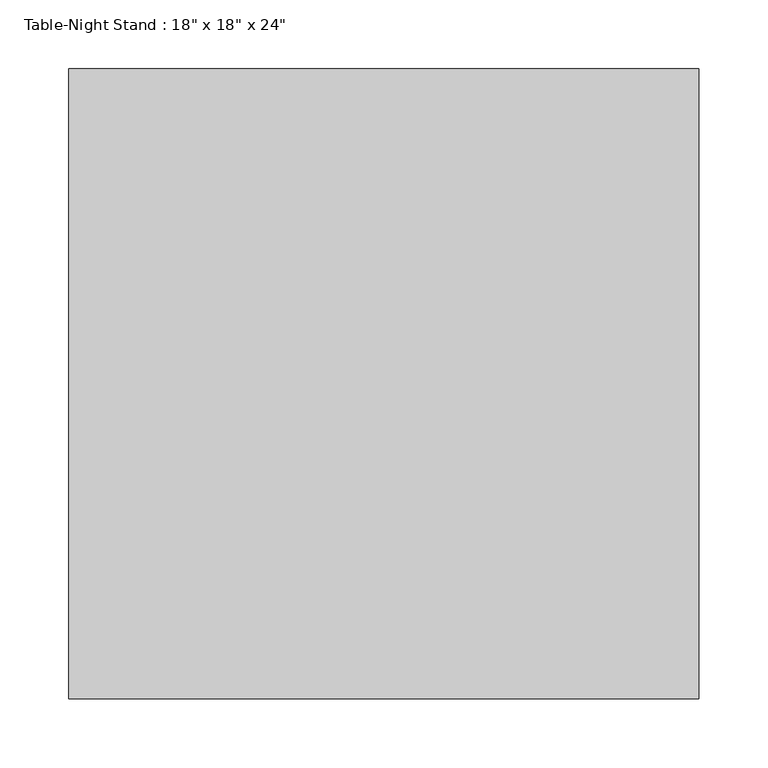
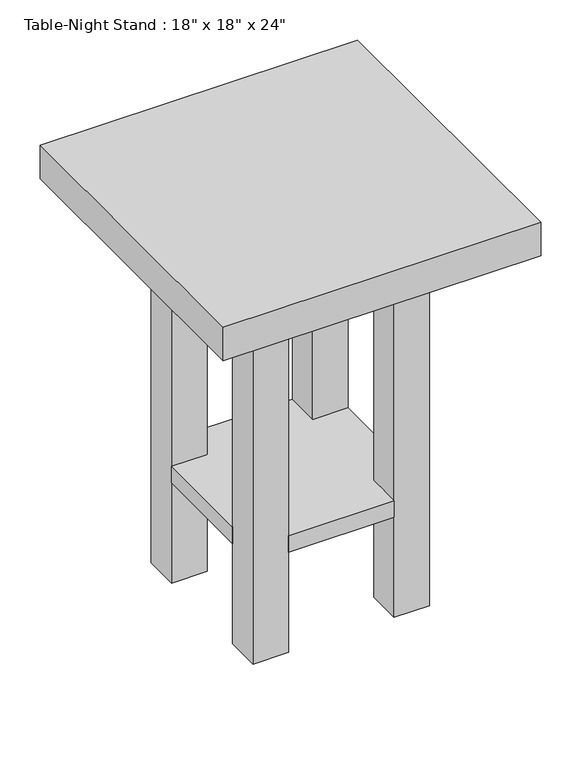
"""IFC4 building model written with IfcOpenShell, lengths in millimetres: furniture geometry."""

import ifcopenshell
import ifcopenshell.guid

model = None  # the IFC model being written
_history = None  # IfcOwnerHistory: only IFC2X3 demands one
_inside = {}  # id of a spatial element -> (the spatial element, [elements in it])
_under = {}  # id of a project, library or spatial element -> (it, [spatial elements below it])
_declared = {}  # id of a project -> (the project, [libraries it declares])
_typed = {}  # id of a type object -> (the type object, [elements of that type])
_made_of = {}  # id of a material, layer set ... -> (it, [elements and type objects made of it])


def new_model(schema):
    """Start an empty IFC model of exactly this schema.

    Asked for "IFC4X3", IfcOpenShell would pick the latest addendum, in which some entities
    have other attributes; the version numbers below select the first issue.
    IFC2X3 requires an IfcOwnerHistory on every rooted entity: one is made here for all.
    """
    global model, _history
    if schema == "IFC4X3":
        model = ifcopenshell.file(schema_version=(4, 3, 0, 0))
    else:
        model = ifcopenshell.file(schema=schema)
    _inside.clear()
    _under.clear()
    _declared.clear()
    _typed.clear()
    _made_of.clear()
    _history = None
    if model.schema == "IFC2X3":
        org = make("IfcOrganization", Name="unknown")
        user = make(
            "IfcPersonAndOrganization",
            ThePerson=make("IfcPerson", FamilyName="unknown"),
            TheOrganization=org,
        )
        app = make(
            "IfcApplication",
            ApplicationDeveloper=org,
            Version="unknown",
            ApplicationFullName="unknown",
            ApplicationIdentifier="unknown",
        )
        _history = make(
            "IfcOwnerHistory",
            OwningUser=user,
            OwningApplication=app,
            ChangeAction="ADDED",
            CreationDate=0,
        )
    return model


def make(cls, **values):
    """One entity of the class cls with the attributes given. An attribute that is None is left unset."""
    return model.create_entity(
        cls, **{name: value for name, value in values.items() if value is not None}
    )


def rooted(cls, **values):
    """An entity with a GlobalId (a new one), such as an element, a storey or a relation."""
    return make(cls, GlobalId=ifcopenshell.guid.new(), OwnerHistory=_history, **values)


def si_unit(unit_type, name, prefix=None):
    """IfcSIUnit, for example si_unit("LENGTHUNIT", "METRE", prefix="MILLI")."""
    return make("IfcSIUnit", UnitType=unit_type, Prefix=prefix, Name=name)


def assignment(units):
    """IfcUnitAssignment: the units of a project."""
    return None if units is None else make("IfcUnitAssignment", Units=units)


def point(xyz):
    """IfcCartesianPoint."""
    return None if xyz is None else make("IfcCartesianPoint", Coordinates=xyz)


def direction(xyz):
    """IfcDirection."""
    return None if xyz is None else make("IfcDirection", DirectionRatios=xyz)


def frame(location, z_axis=None, x_axis=None):
    """IfcAxis2Placement3D, a coordinate frame: its origin and axes. An axis left out is left unset."""
    return make(
        "IfcAxis2Placement3D",
        Location=point(location),
        Axis=direction(z_axis),
        RefDirection=direction(x_axis),
    )


def origin():
    """The frame at (0, 0, 0) with its axes left unset."""
    return frame((0.0, 0.0, 0.0))


def origin_with_axes():
    """The frame at (0, 0, 0) with the z axis (0, 0, 1) and the x axis (1, 0, 0) written out."""
    return frame((0.0, 0.0, 0.0), z_axis=(0.0, 0.0, 1.0), x_axis=(1.0, 0.0, 0.0))


def place(relative_to, where):
    """IfcLocalPlacement: puts the frame where relative to a parent placement (None: the world)."""
    return make(
        "IfcLocalPlacement", PlacementRelTo=relative_to, RelativePlacement=where
    )


def context(
    kind, dimensions, precision=None, world=None, true_north=None, identifier=None
):
    """IfcGeometricRepresentationContext, for example the 3D "Model" context."""
    return make(
        "IfcGeometricRepresentationContext",
        ContextIdentifier=identifier,
        ContextType=kind,
        CoordinateSpaceDimension=dimensions,
        Precision=precision,
        WorldCoordinateSystem=world,
        TrueNorth=true_north,
    )


def project(units=None, contexts=None):
    """IfcProject with its units and contexts."""
    return rooted(
        "IfcProject",
        Name="project",
        RepresentationContexts=contexts,
        UnitsInContext=assignment(units),
    )


def spatial(cls, under=None, at=None, **own):
    """A site, building, storey or space (cls), placed at a placement, below another one or the project."""
    s = rooted(cls, ObjectPlacement=at, **own)
    if under is not None:
        _under.setdefault(under.id(), (under, []))[1].append(s)
    return s


def polyline(points):
    """IfcPolyline through the points."""
    return make("IfcPolyline", Points=[point(p) for p in points])


def outline(outer, holes=None, kind="AREA"):
    """IfcArbitraryClosedProfileDef: a profile drawn as a closed curve; with holes, ...WithVoids."""
    if holes is None:
        return make("IfcArbitraryClosedProfileDef", ProfileType=kind, OuterCurve=outer)
    return make(
        "IfcArbitraryProfileDefWithVoids",
        ProfileType=kind,
        OuterCurve=outer,
        InnerCurves=holes,
    )


def extrude(swept, where, along, depth):
    """IfcExtrudedAreaSolid: the profile swept, set in the frame where, extruded along a direction by depth."""
    return make(
        "IfcExtrudedAreaSolid",
        SweptArea=swept,
        Position=where,
        ExtrudedDirection=direction(along),
        Depth=depth,
    )


def shape(context_of_items, identifier, shape_type, items):
    """IfcShapeRepresentation: the items that make up one representation, for example the "Body"."""
    return make(
        "IfcShapeRepresentation",
        ContextOfItems=context_of_items,
        RepresentationIdentifier=identifier,
        RepresentationType=shape_type,
        Items=items,
    )


def source(mapping_origin, context_of_items, identifier, shape_type, items):
    """IfcRepresentationMap: a shape defined once, which mapped items show again and again."""
    return make(
        "IfcRepresentationMap",
        MappingOrigin=mapping_origin,
        MappedRepresentation=shape(context_of_items, identifier, shape_type, items),
    )


def transform(
    local_origin,
    x_axis=None,
    y_axis=None,
    z_axis=None,
    scale=None,
    scale2=None,
    scale3=None,
    uniform=True,
):
    """IfcCartesianTransformationOperator3D, or its non-uniform kind. x_axis, y_axis, z_axis: its Axis1, 2, 3."""
    if uniform:
        return make(
            "IfcCartesianTransformationOperator3D",
            Axis1=direction(x_axis),
            Axis2=direction(y_axis),
            LocalOrigin=point(local_origin),
            Scale=scale,
            Axis3=direction(z_axis),
        )
    return make(
        "IfcCartesianTransformationOperator3DnonUniform",
        Axis1=direction(x_axis),
        Axis2=direction(y_axis),
        LocalOrigin=point(local_origin),
        Scale=scale,
        Axis3=direction(z_axis),
        Scale2=scale2,
        Scale3=scale3,
    )


def mapped(mapping_source, mapping_target):
    """IfcMappedItem: shows the shape of a source again, moved by a transform."""
    return make(
        "IfcMappedItem", MappingSource=mapping_source, MappingTarget=mapping_target
    )


def made_of(thing, what):
    """Note that an element or type object is made of a material, layer set ...; save() writes the relation."""
    if what is not None:
        _made_of.setdefault(what.id(), (what, []))[1].append(thing)
    return thing


def element(
    cls,
    number,
    at=None,
    inside=None,
    cuts=None,
    type_object=None,
    material=None,
    context=None,
    identifier="Body",
    shape_type=None,
    held_by="IfcProductDefinitionShape",
    body=None,
    shapes=None,
    **own,
):
    """One element of the class cls, such as IfcWall. Its Tag is "e" and its number.

    at: its placement. inside: the storey or other place that contains it. cuts: it is an
    opening in that element (IfcRelVoidsElement). A single representation is given by context,
    identifier, shape_type and body (its items); several are given by shapes. held_by: the class
    of the entity that holds the representations. save() writes the other relations.
    """
    e = rooted(cls, Tag="e%d" % number, ObjectPlacement=at, **own)
    if body is not None:
        shapes = [shape(context, identifier, shape_type, body)]
    if shapes is not None:
        e.Representation = make(held_by, Representations=shapes)
    if inside is not None:
        _inside.setdefault(inside.id(), (inside, []))[1].append(e)
    if cuts is not None:
        rooted(
            "IfcRelVoidsElement", RelatingBuildingElement=cuts, RelatedOpeningElement=e
        )
    if type_object is not None:
        _typed.setdefault(type_object.id(), (type_object, []))[1].append(e)
    return made_of(e, material)


def aggregate(whole, parts):
    """IfcRelAggregates: a whole, such as a stair, and the parts it consists of."""
    return rooted("IfcRelAggregates", RelatingObject=whole, RelatedObjects=parts)


def save(model, path):
    """Write the relations noted so far, then the file.

    IfcRelAggregates (storeys below a building ...), IfcRelContainedInSpatialStructure (elements
    in a storey), IfcRelDefinesByType, IfcRelAssociatesMaterial and IfcRelDeclares: one each for
    every whole, place, type object, material and project.
    """
    for whole, parts in _under.values():
        aggregate(whole, parts)
    for where, things in _inside.values():
        rooted(
            "IfcRelContainedInSpatialStructure",
            RelatedElements=things,
            RelatingStructure=where,
        )
    for kind, things in _typed.values():
        rooted("IfcRelDefinesByType", RelatedObjects=things, RelatingType=kind)
    for what, things in _made_of.values():
        rooted("IfcRelAssociatesMaterial", RelatedObjects=things, RelatingMaterial=what)
    for by, libraries in _declared.values():
        rooted("IfcRelDeclares", RelatingContext=by, RelatedDefinitions=libraries)
    model.write(path)


def furniture_097b63cf(model_context):
    return source(origin(), model_context, "Body", "SweptSolid", [
        extrude(outline(polyline([(156.1336303, 355.6), (308.5336303, 355.6), (308.5336303, 304.8), (359.3336303, 304.8), (359.3336303, 152.4), (308.5336303, 152.4), (308.5336303, 101.6), (156.1336303, 101.6), (156.1336303, 152.4), (105.3336303, 152.4), (105.3336303, 304.8), (156.1336303, 304.8), (156.1336303, 355.6)])), frame((0.0, 0.0, 152.4), z_axis=(0.0, 0.0, 1.0), x_axis=(1.0, 0.0, 0.0)), (0.0, 0.0, 1.0), 25.4),
        extrude(outline(polyline([(156.1336303, 355.6), (156.1336303, 304.8), (105.3336303, 304.8), (105.3336303, 355.6), (156.1336303, 355.6)])), origin_with_axes(), (0.0, 0.0, 1.0), 558.8),
        extrude(outline(polyline([(156.1336303, 152.4), (156.1336303, 101.6), (105.3336303, 101.6), (105.3336303, 152.4), (156.1336303, 152.4)])), origin_with_axes(), (0.0, 0.0, 1.0), 558.8),
        extrude(outline(polyline([(359.3336303, 355.6), (359.3336303, 304.8), (308.5336303, 304.8), (308.5336303, 355.6), (359.3336303, 355.6)])), origin_with_axes(), (0.0, 0.0, 1.0), 558.8),
        extrude(outline(polyline([(359.3336303, 152.4), (359.3336303, 101.6), (308.5336303, 101.6), (308.5336303, 152.4), (359.3336303, 152.4)])), origin_with_axes(), (0.0, 0.0, 1.0), 558.8),
        extrude(outline(polyline([(460.9336303, 0.0), (3.7336303, 0.0), (3.7336303, 457.2), (460.9336303, 457.2), (460.9336303, 0.0)])), frame((0.0, 0.0, 558.8), z_axis=(0.0, 0.0, 1.0), x_axis=(1.0, 0.0, 0.0)), (0.0, 0.0, 1.0), 50.8),
    ])


if __name__ == "__main__":
    model = new_model("IFC4")
    model_context = context("Model", 3, world=origin())
    ifc_project = project(units=[si_unit("LENGTHUNIT", "METRE", prefix="MILLI")], contexts=[model_context])
    site = spatial("IfcSite", under=ifc_project)
    building = spatial("IfcBuilding", under=site)
    placement = place(None, origin())
    furniture_shape = furniture_097b63cf(model_context)
    element("IfcFurniture", 1, ObjectType="Table-Night Stand : 18\" x 18\" x 24\"", at=placement, inside=building, context=model_context, shape_type="MappedRepresentation", body=[
        mapped(furniture_shape, transform((0.0, 0.0, 0.0), x_axis=(1.0, 0.0, 0.0), y_axis=(0.0, 1.0, 0.0), z_axis=(0.0, 0.0, 1.0))),
    ])
    save(model, "model.ifc")

# Revit data of these elements
# Project information
#   Project Issue Date = "Issue Date"
#   Project Status = "Project Status"
#   Client Name = "Owner"
#   Project Address = "Enter address here"
#   Project Name = "Project Name"
#   Project Number = "Project Number"
# Type "Table-Night Stand : 18\" x 18\" x 24\""
#   Assembly Code = "E2020200"
#   Depth = 1' - 6"
#   Height = 2' - 0"
#   Width = 1' - 6"
#   Base Material = Birch
#   Top Material = Laminate, Ivory, Matte
# Element 1 (IfcFurniture, "Table-Night Stand : 18\" x 18\" x 24\"")
#   Materials on its faces: "Birch", "Laminate, Ivory, Matte"
# Materials
#   "Birch": class "Wood", colour RGB 224 178 126, transparency 0, Description = "Betula Alleghaniensis", Cost = 0
#   "Laminate, Ivory, Matte": class "Plastic", colour RGB 247 247 239, transparency 0, Description = "Plastic Laminate - Ivory, Matte", Cost = 0
